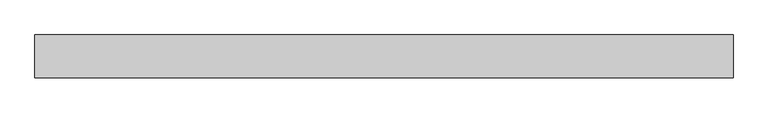
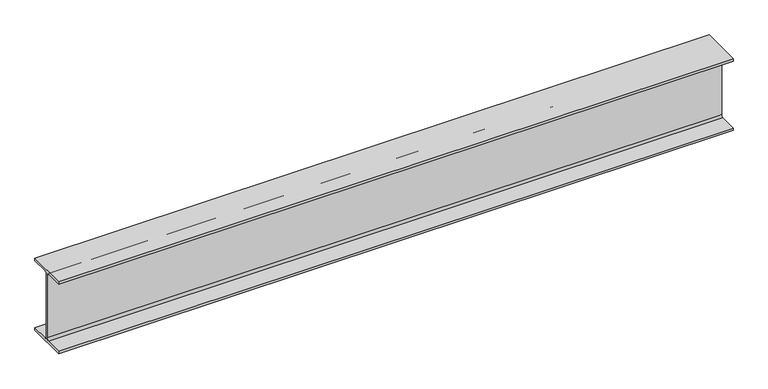
"""IFC4 building model written with IfcOpenShell, lengths in millimetres: beam geometry, Old_Steel Beam_H-KSD3502 : H_SB_ASB_H-194×150x6x9."""

from ifc_helpers import new_model, si_unit, point, frame, frame_2d, origin, place, context, project, spatial, polyline, circle_curve, trimmed, segment, composite_curve, outline, extrude, source, transform, mapped, element, save


def beam_172751ac(model_context):
    return source(origin(), model_context, "Body", "SweptSolid", [
        extrude(outline(composite_curve([segment(polyline([(-82.5, -141.5), (-11.9, -141.5)]), True, "CONTINUOUS"), segment(trimmed(circle_curve(frame_2d((-11.9, -132.6)), 8.9), [point((-11.9, -141.5))], [point((-3.0, -132.6))], True, "CARTESIAN"), True, "CONTINUOUS"), segment(polyline([(-3.0, -132.6), (-3.0, 132.6)]), True, "CONTINUOUS"), segment(trimmed(circle_curve(frame_2d((-11.9, 132.6)), 8.9), [point((-3.0, 132.6))], [point((-11.9, 141.5))], True, "CARTESIAN"), True, "CONTINUOUS"), segment(polyline([(-11.9, 141.5), (-82.5, 141.5), (-82.5, 151.7), (82.5, 151.7), (82.5, 141.5), (11.9, 141.5)]), True, "CONTINUOUS"), segment(trimmed(circle_curve(frame_2d((11.9, 132.6)), 8.9), [point((11.9, 141.5))], [point((3.0, 132.6))], True, "CARTESIAN"), True, "CONTINUOUS"), segment(polyline([(3.0, 132.6), (3.0, -132.6)]), True, "CONTINUOUS"), segment(trimmed(circle_curve(frame_2d((11.9, -132.6)), 8.9), [point((3.0, -132.6))], [point((11.9, -141.5))], True, "CARTESIAN"), True, "CONTINUOUS"), segment(polyline([(11.9, -141.5), (82.5, -141.5), (82.5, -151.7), (-82.5, -151.7), (-82.5, -141.5)]), True, "CONTINUOUS")], self_intersect=False)), frame((-1200.1295083, 0.0, 0.0), z_axis=(1.0, 0.0, 0.0), x_axis=(0.0, 1.0, 0.0)), (0.0, 0.0, 1.0), 2693.3121073),
    ])


if __name__ == "__main__":
    model = new_model("IFC4")
    model_context = context("Model", 3, world=origin())
    ifc_project = project(units=[si_unit("LENGTHUNIT", "METRE", prefix="MILLI")], contexts=[model_context])
    site = spatial("IfcSite", under=ifc_project)
    building = spatial("IfcBuilding", under=site)
    placement = place(None, origin())
    beam_shape = beam_172751ac(model_context)
    element("IfcBeam", 1, ObjectType="Old_Steel Beam_H-KSD3502 : H_SB_ASB_H-194×150x6x9", at=placement, inside=building, context=model_context, shape_type="MappedRepresentation", body=[
        mapped(beam_shape, transform((0.0, 0.0, 0.0), x_axis=(1.0, 0.0, 0.0), y_axis=(0.0, 1.0, 0.0), z_axis=(0.0, 0.0, 1.0))),
    ])
    save(model, "model.ifc")

# Revit data of these elements
# Type "Old_Steel Beam_H-KSD3502 : H_SB_ASB_H-194×150x6x9"
#   Width = 15.0 cm
#   Web Thickness = 0.6 cm
#   Web Fillet = 1.3 cm
#   Warping Constant = 43316.0 cm⁶
#   Torsional Moment of Inertia = 8.622 cm⁴
#   Torsional Modulus = 1.0 cm³
#   Section Area = 39.01 cm²
#   Plastic Modulus weak axis = 104.0 cm³
#   Plastic Modulus strong axis = 309.0 cm³
#   Perimeter = 0.95 m²/m
#   Nominal Weight = 30.60 kgf/m
#   Moment of Inertia weak axis = 507.00 cm⁴
#   Moment of Inertia strong axis = 2690.00 cm⁴
#   Height = 19.4 cm
#   Flange Thickness = 0.9 cm
#   Elastic Modulus weak axis = 67.6 cm³
#   Elastic Modulus strong axis = 277.0 cm³
#   Centroid Vertical = 9.7 cm
#   Centroid Horizontal = 7.5 cm
#   Length [instance default] = 1.5240 m
#   Structural Material [instance default] = Steel, 45-345
#   Assembly Code = ""
# Element 1 (IfcBeam, "Old_Steel Beam_H-KSD3502 : H_SB_ASB_H-194×150x6x9")
#   Structural Material = none
# Materials
#   "Steel, 45-345": class "Metal", colour RGB 189 187 185, transparency 0, Description = "Steel 345 MPa", Cost = 0
